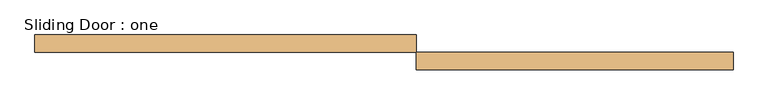
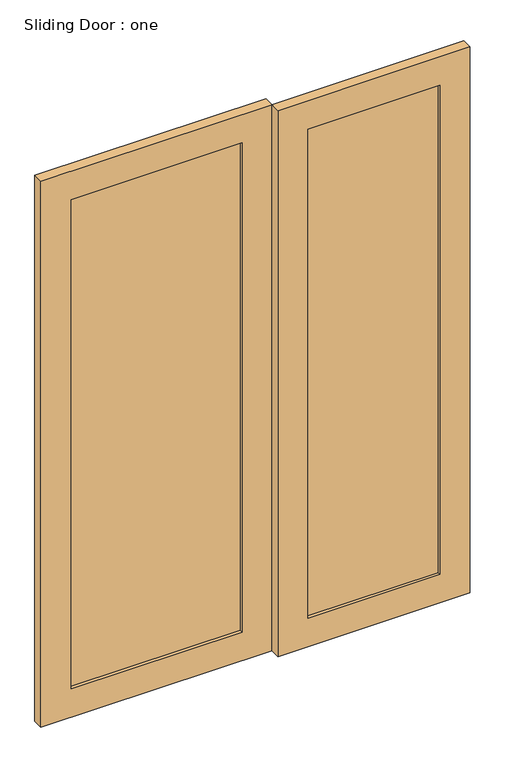
"""IFC4 building model written with IfcOpenShell, lengths in millimetres: door geometry, Sliding Door : one."""

from ifc_helpers import new_model, si_unit, frame, origin, place, context, project, spatial, polyline, outline, extrude, source, transform, mapped, element, save


def sliding_door_one_977cb0c7(model_context):
    return source(origin(), model_context, "Body", "SweptSolid", [
        extrude(outline(polyline([(-44.4768999, 50.8), (-44.4768999, 31.75), (-766.7625, 31.75), (-766.7625, 50.8), (-44.4768999, 50.8)])), frame((0.0, 0.0, 127.0), z_axis=(0.0, 0.0, 1.0), x_axis=(1.0, 0.0, 0.0)), (0.0, 0.0, 1.0), 2184.4),
        extrude(outline(polyline([(766.7625, 6.35), (766.7625, -12.7), (209.5231001, -12.7), (209.5231001, 6.35), (766.7625, 6.35)])), frame((0.0, 0.0, 127.0), z_axis=(0.0, 0.0, 1.0), x_axis=(1.0, 0.0, 0.0)), (0.0, 0.0, 1.0), 2184.4),
        extrude(outline(polyline([(2438.4, -893.7625), (0.0, -893.7625), (0.0, 82.5231001), (2438.4, 82.5231001), (2438.4, -893.7625)]), holes=[polyline([(127.0, -44.4768999), (127.0, -766.7625), (2311.4, -766.7625), (2311.4, -44.4768999), (127.0, -44.4768999)])]), frame((0.0, 19.05, 0.0), z_axis=(0.0, 1.0, 0.0), x_axis=(0.0, 0.0, 1.0)), (0.0, 0.0, 1.0), 44.45),
        extrude(outline(polyline([(2438.4, 82.5231001), (0.0, 82.5231001), (0.0, 893.7625), (2438.4, 893.7625), (2438.4, 82.5231001)]), holes=[polyline([(127.0, 766.7625), (127.0, 209.5231001), (2311.4, 209.5231001), (2311.4, 766.7625), (127.0, 766.7625)])]), frame((0.0, -25.4, 0.0), z_axis=(0.0, 1.0, 0.0), x_axis=(0.0, 0.0, 1.0)), (0.0, 0.0, 1.0), 44.45),
    ])


if __name__ == "__main__":
    model = new_model("IFC4")
    model_context = context("Model", 3, world=origin())
    ifc_project = project(units=[si_unit("LENGTHUNIT", "METRE", prefix="MILLI")], contexts=[model_context])
    site = spatial("IfcSite", under=ifc_project)
    building = spatial("IfcBuilding", under=site)
    placement = place(None, origin())
    sliding_door_one_shape = sliding_door_one_977cb0c7(model_context)
    element("IfcDoor", 1, ObjectType="Sliding Door : one", at=placement, inside=building, context=model_context, shape_type="MappedRepresentation", body=[
        mapped(sliding_door_one_shape, transform((0.0, 0.0, 0.0), x_axis=(1.0, 0.0, 0.0), y_axis=(0.0, 1.0, 0.0), z_axis=(0.0, 0.0, 1.0))),
    ])
    save(model, "model.ifc")

# Revit data of these elements
# Type "Sliding Door : one"
#   Type Mark = "42"
#   Analytic Construction = "<None>"
#   Stile_Width = 0' - 5"
#   Door_Thickness = 0' - 1 3/4"
#   Door_Offset = 0' - 1"
#   Glass_Material = SAFETY GLAZING
#   Frame_Material = INTERIOR GRADE ALUMINUM STOREFRONT W/ SAFETY GLAZING
#   Function = (empty or 0)
# Element 1 (IfcDoor, "Sliding Door : one")
#   Materials on its faces: "INTERIOR GRADE ALUMINUM STOREFRONT W/ SAFETY GLAZING", "SAFETY GLAZING"
# Materials
#   "SAFETY GLAZING": class "Glass", colour RGB 142 168 196, transparency 0.75, Description = "Soda Lime Glass", Cost = 0
#   "INTERIOR GRADE ALUMINUM STOREFRONT W/ SAFETY GLAZING": class "Metal", colour RGB 226 226 226, transparency 0, Description = "Aluminum 6061", Cost = 0
